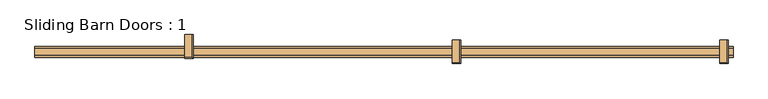
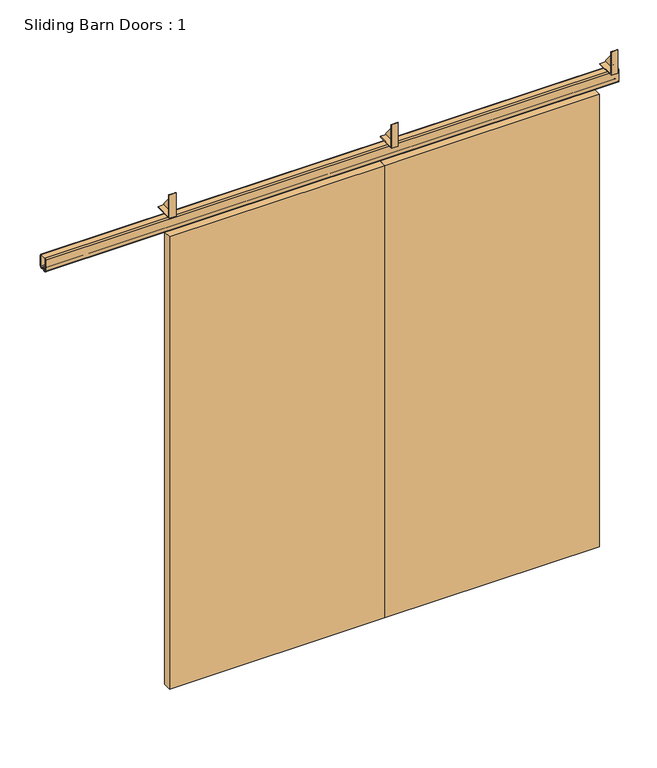
"""IFC4 building model written with IfcOpenShell, lengths in millimetres: door geometry, Sliding Barn Doors : 1."""

from ifc_helpers import new_model, si_unit, point, frame, frame_2d, origin, place, context, project, spatial, polyline, circle_curve, trimmed, segment, composite_curve, outline, extrude, source, transform, mapped, element, save


def sliding_barn_doors_1_1ad96ae7(model_context):
    return source(origin(), model_context, "Body", "SweptSolid", [
        extrude(outline(polyline([(158.75, 2152.65), (158.75, 2146.3), (79.375, 2146.3), (79.375, 2247.773), (158.75, 2152.65)])), frame((-1418.4808594, 0.0, 0.0), z_axis=(1.0, 0.0, 0.0), x_axis=(0.0, 1.0, 0.0)), (0.0, 0.0, 1.0), 3.175),
        extrude(outline(polyline([(76.2, 2143.125), (76.2, 2247.773), (79.375, 2247.773), (79.375, 2146.3), (158.75, 2146.3), (158.75, 2143.125), (76.2, 2143.125)])), frame((-1443.7816406, 0.0, 0.0), z_axis=(1.0, 0.0, 0.0), x_axis=(0.0, 1.0, 0.0)), (0.0, 0.0, 1.0), 28.4757812),
        extrude(outline(polyline([(139.7, 2152.65), (139.7, 2146.3), (60.325, 2146.3), (60.325, 2247.773), (139.7, 2152.65)])), frame((-484.2371094, 0.0, 0.0), z_axis=(1.0, 0.0, 0.0), x_axis=(0.0, 1.0, 0.0)), (0.0, 0.0, 1.0), 3.175),
        extrude(outline(polyline([(57.15, 2143.125), (57.15, 2247.773), (60.325, 2247.773), (60.325, 2146.3), (139.7, 2146.3), (139.7, 2143.125), (57.15, 2143.125)])), frame((-509.5378906, 0.0, 0.0), z_axis=(1.0, 0.0, 0.0), x_axis=(0.0, 1.0, 0.0)), (0.0, 0.0, 1.0), 28.4757813),
        extrude(outline(polyline([(139.7, 2152.65), (139.7, 2146.3), (60.325, 2146.3), (60.325, 2247.773), (139.7, 2152.65)])), frame((450.0066406, 0.0, 0.0), z_axis=(1.0, 0.0, 0.0), x_axis=(0.0, 1.0, 0.0)), (0.0, 0.0, 1.0), 3.175),
        extrude(outline(polyline([(57.15, 2143.125), (57.15, 2247.773), (60.325, 2247.773), (60.325, 2146.3), (139.7, 2146.3), (139.7, 2143.125), (57.15, 2143.125)])), frame((424.7058594, 0.0, 0.0), z_axis=(1.0, 0.0, 0.0), x_axis=(0.0, 1.0, 0.0)), (0.0, 0.0, 1.0), 28.4757813),
        extrude(outline(polyline([(-1339.31025, 117.475), (-1288.00225, 117.475), (-1288.00225, 114.3), (-1339.31025, 114.3), (-1339.31025, 117.475)])), frame((0.0, 0.0, 1889.252), z_axis=(0.0, 0.0, 1.0), x_axis=(1.0, 0.0, 0.0)), (0.0, 0.0, 1.0), 168.148),
        extrude(outline(polyline([(-678.91025, 117.475), (-627.60225, 117.475), (-627.60225, 114.3), (-678.91025, 114.3), (-678.91025, 117.475)])), frame((0.0, 0.0, 1889.252), z_axis=(0.0, 0.0, 1.0), x_axis=(1.0, 0.0, 0.0)), (0.0, 0.0, 1.0), 168.148),
        extrude(outline(polyline([(-424.91025, 117.475), (-373.60225, 117.475), (-373.60225, 114.3), (-424.91025, 114.3), (-424.91025, 117.475)])), frame((0.0, 0.0, 1889.252), z_axis=(0.0, 0.0, 1.0), x_axis=(1.0, 0.0, 0.0)), (0.0, 0.0, 1.0), 168.148),
        extrude(outline(polyline([(235.48975, 117.475), (286.79775, 117.475), (286.79775, 114.3), (235.48975, 114.3), (235.48975, 117.475)])), frame((0.0, 0.0, 1889.252), z_axis=(0.0, 0.0, 1.0), x_axis=(1.0, 0.0, 0.0)), (0.0, 0.0, 1.0), 168.148),
        extrude(outline(polyline([(-1440.65625, 114.3), (-526.25625, 114.3), (-526.25625, 79.375), (-1440.65625, 79.375), (-1440.65625, 114.3)])), frame((0.0, 0.0, 25.4), z_axis=(0.0, 0.0, 1.0), x_axis=(1.0, 0.0, 0.0)), (0.0, 0.0, 1.0), 2032.0),
        extrude(outline(polyline([(-526.25625, 114.3), (388.14375, 114.3), (388.14375, 79.375), (-526.25625, 79.375), (-526.25625, 114.3)])), frame((0.0, 0.0, 25.4), z_axis=(0.0, 0.0, 1.0), x_axis=(1.0, 0.0, 0.0)), (0.0, 0.0, 1.0), 2032.0),
        extrude(outline(composite_curve([segment(polyline([(85.725, 2143.125), (111.252, 2143.125)]), True, "CONTINUOUS"), segment(trimmed(circle_curve(frame_2d((111.252, 2136.775)), 6.35), [point((111.252, 2143.125))], [point((117.602, 2136.775))], False, "CARTESIAN"), True, "CONTINUOUS"), segment(polyline([(117.602, 2136.775), (117.602, 2088.515)]), True, "CONTINUOUS"), segment(trimmed(circle_curve(frame_2d((111.252, 2088.515)), 6.35), [point((117.602, 2088.515))], [point((111.252, 2082.165))], False, "CARTESIAN"), True, "CONTINUOUS"), segment(polyline([(111.252, 2082.165), (105.8433147, 2082.165)]), True, "CONTINUOUS"), segment(trimmed(circle_curve(frame_2d((105.8433147, 2083.7525)), 1.5875), [point((105.8433147, 2082.165))], [point((104.2849816, 2083.4495907))], False, "CARTESIAN"), True, "CONTINUOUS"), segment(polyline([(104.2849816, 2083.4495907), (102.8594659, 2090.7832331), (104.3756029, 2090.7832331), (105.7615251, 2083.6532812), (111.252, 2083.6532812)]), True, "CONTINUOUS"), segment(trimmed(circle_curve(frame_2d((111.252, 2088.515)), 4.8617187), [point((111.252, 2083.6532812))], [point((116.1137188, 2088.515))], True, "CARTESIAN"), True, "CONTINUOUS"), segment(polyline([(116.1137188, 2088.515), (116.1137188, 2136.775)]), True, "CONTINUOUS"), segment(trimmed(circle_curve(frame_2d((111.252, 2136.775)), 4.8617187), [point((116.1137188, 2136.775))], [point((111.252, 2141.6367187))], True, "CARTESIAN"), True, "CONTINUOUS"), segment(polyline([(111.252, 2141.6367187), (85.725, 2141.6367187)]), True, "CONTINUOUS"), segment(trimmed(circle_curve(frame_2d((85.725, 2136.775)), 4.8617187), [point((85.725, 2141.6367187))], [point((80.8632813, 2136.775))], True, "CARTESIAN"), True, "CONTINUOUS"), segment(polyline([(80.8632813, 2136.775), (80.8632813, 2088.515)]), True, "CONTINUOUS"), segment(trimmed(circle_curve(frame_2d((85.725, 2088.515)), 4.8617187), [point((80.8632813, 2088.515))], [point((85.725, 2083.6532812))], True, "CARTESIAN"), True, "CONTINUOUS"), segment(polyline([(85.725, 2083.6532812), (91.2154749, 2083.6532812), (92.6013971, 2090.7832331), (94.1175341, 2090.7832331), (92.6920184, 2083.4495907)]), True, "CONTINUOUS"), segment(trimmed(circle_curve(frame_2d((91.1336853, 2083.7525)), 1.5875), [point((92.6920184, 2083.4495907))], [point((91.1336853, 2082.165))], False, "CARTESIAN"), True, "CONTINUOUS"), segment(polyline([(91.1336853, 2082.165), (85.725, 2082.165)]), True, "CONTINUOUS"), segment(trimmed(circle_curve(frame_2d((85.725, 2088.515)), 6.35), [point((85.725, 2082.165))], [point((79.375, 2088.515))], False, "CARTESIAN"), True, "CONTINUOUS"), segment(polyline([(79.375, 2088.515), (79.375, 2136.775)]), True, "CONTINUOUS"), segment(trimmed(circle_curve(frame_2d((85.725, 2136.775)), 6.35), [point((79.375, 2136.775))], [point((85.725, 2143.125))], False, "CARTESIAN"), True, "CONTINUOUS")], self_intersect=False)), frame((-1967.70625, 0.0, 0.0), z_axis=(1.0, 0.0, 0.0), x_axis=(0.0, 1.0, 0.0)), (0.0, 0.0, 1.0), 2438.4),
    ])


if __name__ == "__main__":
    model = new_model("IFC4")
    model_context = context("Model", 3, world=origin())
    ifc_project = project(units=[si_unit("LENGTHUNIT", "METRE", prefix="MILLI")], contexts=[model_context])
    site = spatial("IfcSite", under=ifc_project)
    building = spatial("IfcBuilding", under=site)
    placement = place(None, origin())
    sliding_barn_doors_1_shape = sliding_barn_doors_1_1ad96ae7(model_context)
    element("IfcDoor", 1, ObjectType="Sliding Barn Doors : 1", at=placement, inside=building, context=model_context, shape_type="MappedRepresentation", body=[
        mapped(sliding_barn_doors_1_shape, transform((0.0, 0.0, 0.0), x_axis=(1.0, 0.0, 0.0), y_axis=(0.0, 1.0, 0.0), z_axis=(0.0, 0.0, 1.0))),
    ])
    save(model, "model.ifc")

# Revit data of these elements
# Type "Sliding Barn Doors : 1"
#   Type Mark = "26"
#   OD_DS_Door_Material = "T.B.D."
#   OD_DS_Door_Type = "SLIDER"
#   OD_DS_Lockset = "-"
#   Analytic Construction = "<None>"
#   rail_overlap_left = 0' - 5 1/4"
#   rail_length = 8' - 0"
#   overlap_left = 0' - 2"
#   overlap = 0' - 0"
#   bracket_right = 3' - 7"
#   bracket_left = 0' - 4"
#   Thickness = 0' - 1 3/8"
#   Panel Width = 3' - 0"
#   Panel Height = 6' - 8"
#   Gap 2 = 0' - 0 1/2"
#   Gap 1 = 0' - 0 7/8"
#   Frame Projection Ext. = 0' - 1"
#   Frame Projection Int. = 0' - 1"
#   Frame Width = 0' - 3"
#   Height = 6' - 4"
#   Width = 2' - 2 9/16"
#   Bracket_offset = 0' - 5"
#   Door_4 = no
#   Door_3 = no
#   Hardware Material = Metal - Aluminum
#   Door Material = Closet_1
#   Function = (empty or 0)
#   Wall Closure = (empty or 0)
# Element 1 (IfcDoor, "Sliding Barn Doors : 1")
#   Materials on its faces: "Metal - Aluminum", "Closet_1"
# Materials
#   "Metal - Aluminum": class "Metal", colour RGB 247 247 247, transparency 0
#   "Closet_1": class "Paint", colour RGB 200 194 183, transparency 0, Cost = 0
